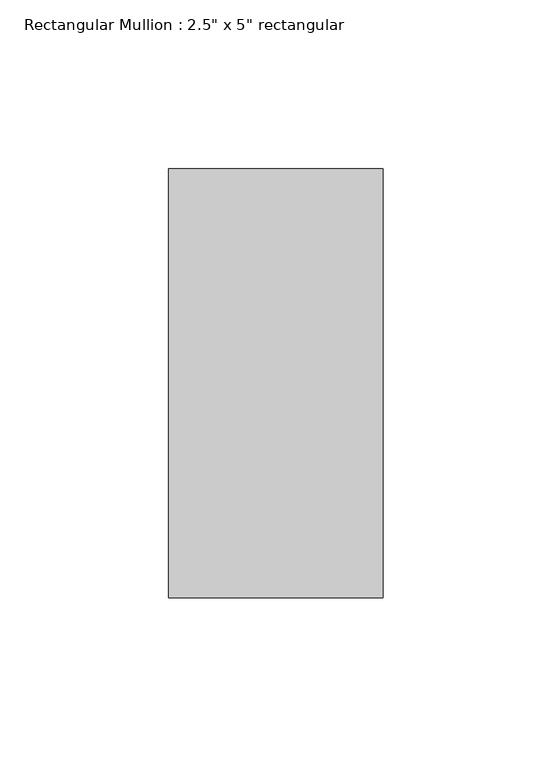
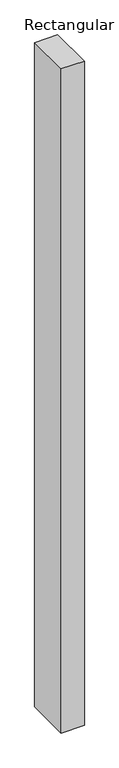
"""IFC4 building model written with IfcOpenShell, lengths in millimetres: member geometry."""

from ifc_helpers import new_model, si_unit, frame, origin, place, context, project, spatial, polyline, outline, extrude, source, transform, mapped, element, save


def member_4f18b2ac(model_context):
    return source(origin(), model_context, "Body", "SweptSolid", [
        extrude(outline(polyline([(0.0, 63.5), (0.0, -63.5), (-63.5, -63.5), (-63.5, 63.5), (0.0, 63.5)])), frame((0.0, 0.0, -1936.75), z_axis=(0.0, 0.0, 1.0), x_axis=(1.0, 0.0, 0.0)), (0.0, 0.0, 1.0), 1936.75),
    ])


if __name__ == "__main__":
    model = new_model("IFC4")
    model_context = context("Model", 3, world=origin())
    ifc_project = project(units=[si_unit("LENGTHUNIT", "METRE", prefix="MILLI")], contexts=[model_context])
    site = spatial("IfcSite", under=ifc_project)
    building = spatial("IfcBuilding", under=site)
    placement = place(None, origin())
    member_shape = member_4f18b2ac(model_context)
    element("IfcMember", 1, ObjectType="Rectangular Mullion : 2.5\" x 5\" rectangular", at=placement, inside=building, context=model_context, shape_type="MappedRepresentation", body=[
        mapped(member_shape, transform((0.0, 0.0, 0.0), x_axis=(1.0, 0.0, 0.0), y_axis=(0.0, 1.0, 0.0), z_axis=(0.0, 0.0, 1.0))),
    ])
    save(model, "model.ifc")

# Revit data of these elements
# Type "Rectangular Mullion : 2.5\" x 5\" rectangular"
#   built-in parameter 1007304 = 0.416667 (stored number, unit not read)
#   built-in parameter 1007301 = 0.104167 (stored number, unit not read)
#   built-in parameter 1007300 = 0.104167 (stored number, unit not read)
# Element 1 (IfcMember, "Rectangular Mullion : 2.5\" x 5\" rectangular")
#   Materials on its faces: "Metal - Aluminum"
# Materials
#   "Metal - Aluminum": class "Metal", colour RGB 140 140 140, transparency 0
